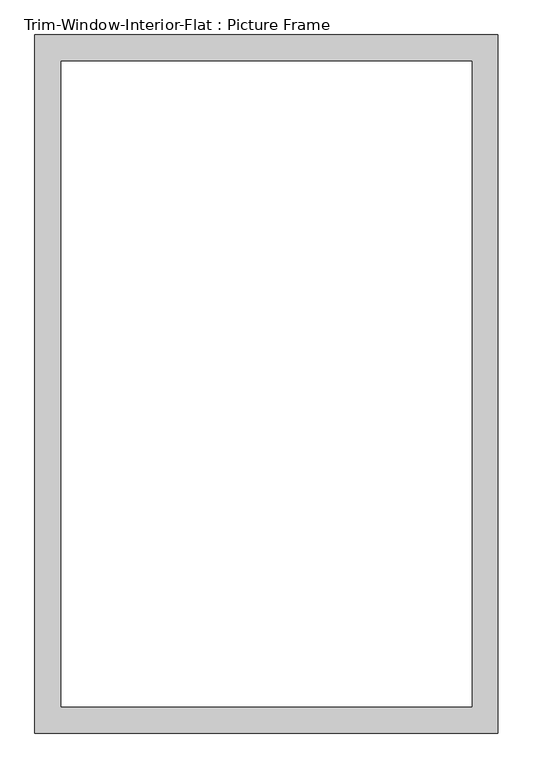
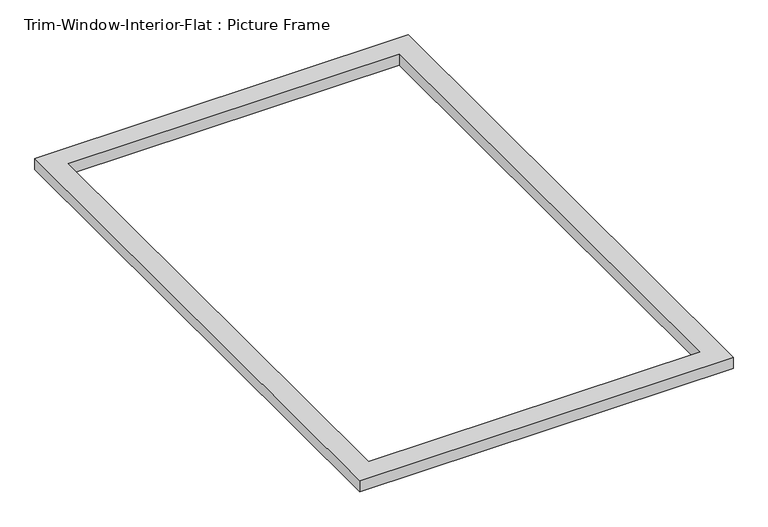
"""IFC4 building model written with IfcOpenShell, lengths in millimetres: proxy geometry, Trim-Window-Interior-Flat : Picture Frame."""

import ifcopenshell
import ifcopenshell.guid

model = None  # the IFC model being written
_history = None  # IfcOwnerHistory: only IFC2X3 demands one
_inside = {}  # id of a spatial element -> (the spatial element, [elements in it])
_under = {}  # id of a project, library or spatial element -> (it, [spatial elements below it])
_declared = {}  # id of a project -> (the project, [libraries it declares])
_typed = {}  # id of a type object -> (the type object, [elements of that type])
_made_of = {}  # id of a material, layer set ... -> (it, [elements and type objects made of it])


def new_model(schema):
    """Start an empty IFC model of exactly this schema.

    Asked for "IFC4X3", IfcOpenShell would pick the latest addendum, in which some entities
    have other attributes; the version numbers below select the first issue.
    IFC2X3 requires an IfcOwnerHistory on every rooted entity: one is made here for all.
    """
    global model, _history
    if schema == "IFC4X3":
        model = ifcopenshell.file(schema_version=(4, 3, 0, 0))
    else:
        model = ifcopenshell.file(schema=schema)
    _inside.clear()
    _under.clear()
    _declared.clear()
    _typed.clear()
    _made_of.clear()
    _history = None
    if model.schema == "IFC2X3":
        org = make("IfcOrganization", Name="unknown")
        user = make(
            "IfcPersonAndOrganization",
            ThePerson=make("IfcPerson", FamilyName="unknown"),
            TheOrganization=org,
        )
        app = make(
            "IfcApplication",
            ApplicationDeveloper=org,
            Version="unknown",
            ApplicationFullName="unknown",
            ApplicationIdentifier="unknown",
        )
        _history = make(
            "IfcOwnerHistory",
            OwningUser=user,
            OwningApplication=app,
            ChangeAction="ADDED",
            CreationDate=0,
        )
    return model


def make(cls, **values):
    """One entity of the class cls with the attributes given. An attribute that is None is left unset."""
    return model.create_entity(
        cls, **{name: value for name, value in values.items() if value is not None}
    )


def rooted(cls, **values):
    """An entity with a GlobalId (a new one), such as an element, a storey or a relation."""
    return make(cls, GlobalId=ifcopenshell.guid.new(), OwnerHistory=_history, **values)


def si_unit(unit_type, name, prefix=None):
    """IfcSIUnit, for example si_unit("LENGTHUNIT", "METRE", prefix="MILLI")."""
    return make("IfcSIUnit", UnitType=unit_type, Prefix=prefix, Name=name)


def assignment(units):
    """IfcUnitAssignment: the units of a project."""
    return None if units is None else make("IfcUnitAssignment", Units=units)


def point(xyz):
    """IfcCartesianPoint."""
    return None if xyz is None else make("IfcCartesianPoint", Coordinates=xyz)


def direction(xyz):
    """IfcDirection."""
    return None if xyz is None else make("IfcDirection", DirectionRatios=xyz)


def frame(location, z_axis=None, x_axis=None):
    """IfcAxis2Placement3D, a coordinate frame: its origin and axes. An axis left out is left unset."""
    return make(
        "IfcAxis2Placement3D",
        Location=point(location),
        Axis=direction(z_axis),
        RefDirection=direction(x_axis),
    )


def origin():
    """The frame at (0, 0, 0) with its axes left unset."""
    return frame((0.0, 0.0, 0.0))


def origin_with_axes():
    """The frame at (0, 0, 0) with the z axis (0, 0, 1) and the x axis (1, 0, 0) written out."""
    return frame((0.0, 0.0, 0.0), z_axis=(0.0, 0.0, 1.0), x_axis=(1.0, 0.0, 0.0))


def place(relative_to, where):
    """IfcLocalPlacement: puts the frame where relative to a parent placement (None: the world)."""
    return make(
        "IfcLocalPlacement", PlacementRelTo=relative_to, RelativePlacement=where
    )


def context(
    kind, dimensions, precision=None, world=None, true_north=None, identifier=None
):
    """IfcGeometricRepresentationContext, for example the 3D "Model" context."""
    return make(
        "IfcGeometricRepresentationContext",
        ContextIdentifier=identifier,
        ContextType=kind,
        CoordinateSpaceDimension=dimensions,
        Precision=precision,
        WorldCoordinateSystem=world,
        TrueNorth=true_north,
    )


def project(units=None, contexts=None):
    """IfcProject with its units and contexts."""
    return rooted(
        "IfcProject",
        Name="project",
        RepresentationContexts=contexts,
        UnitsInContext=assignment(units),
    )


def spatial(cls, under=None, at=None, **own):
    """A site, building, storey or space (cls), placed at a placement, below another one or the project."""
    s = rooted(cls, ObjectPlacement=at, **own)
    if under is not None:
        _under.setdefault(under.id(), (under, []))[1].append(s)
    return s


def polyline(points):
    """IfcPolyline through the points."""
    return make("IfcPolyline", Points=[point(p) for p in points])


def outline(outer, holes=None, kind="AREA"):
    """IfcArbitraryClosedProfileDef: a profile drawn as a closed curve; with holes, ...WithVoids."""
    if holes is None:
        return make("IfcArbitraryClosedProfileDef", ProfileType=kind, OuterCurve=outer)
    return make(
        "IfcArbitraryProfileDefWithVoids",
        ProfileType=kind,
        OuterCurve=outer,
        InnerCurves=holes,
    )


def extrude(swept, where, along, depth):
    """IfcExtrudedAreaSolid: the profile swept, set in the frame where, extruded along a direction by depth."""
    return make(
        "IfcExtrudedAreaSolid",
        SweptArea=swept,
        Position=where,
        ExtrudedDirection=direction(along),
        Depth=depth,
    )


def shape(context_of_items, identifier, shape_type, items):
    """IfcShapeRepresentation: the items that make up one representation, for example the "Body"."""
    return make(
        "IfcShapeRepresentation",
        ContextOfItems=context_of_items,
        RepresentationIdentifier=identifier,
        RepresentationType=shape_type,
        Items=items,
    )


def source(mapping_origin, context_of_items, identifier, shape_type, items):
    """IfcRepresentationMap: a shape defined once, which mapped items show again and again."""
    return make(
        "IfcRepresentationMap",
        MappingOrigin=mapping_origin,
        MappedRepresentation=shape(context_of_items, identifier, shape_type, items),
    )


def transform(
    local_origin,
    x_axis=None,
    y_axis=None,
    z_axis=None,
    scale=None,
    scale2=None,
    scale3=None,
    uniform=True,
):
    """IfcCartesianTransformationOperator3D, or its non-uniform kind. x_axis, y_axis, z_axis: its Axis1, 2, 3."""
    if uniform:
        return make(
            "IfcCartesianTransformationOperator3D",
            Axis1=direction(x_axis),
            Axis2=direction(y_axis),
            LocalOrigin=point(local_origin),
            Scale=scale,
            Axis3=direction(z_axis),
        )
    return make(
        "IfcCartesianTransformationOperator3DnonUniform",
        Axis1=direction(x_axis),
        Axis2=direction(y_axis),
        LocalOrigin=point(local_origin),
        Scale=scale,
        Axis3=direction(z_axis),
        Scale2=scale2,
        Scale3=scale3,
    )


def mapped(mapping_source, mapping_target):
    """IfcMappedItem: shows the shape of a source again, moved by a transform."""
    return make(
        "IfcMappedItem", MappingSource=mapping_source, MappingTarget=mapping_target
    )


def made_of(thing, what):
    """Note that an element or type object is made of a material, layer set ...; save() writes the relation."""
    if what is not None:
        _made_of.setdefault(what.id(), (what, []))[1].append(thing)
    return thing


def element(
    cls,
    number,
    at=None,
    inside=None,
    cuts=None,
    type_object=None,
    material=None,
    context=None,
    identifier="Body",
    shape_type=None,
    held_by="IfcProductDefinitionShape",
    body=None,
    shapes=None,
    **own,
):
    """One element of the class cls, such as IfcWall. Its Tag is "e" and its number.

    at: its placement. inside: the storey or other place that contains it. cuts: it is an
    opening in that element (IfcRelVoidsElement). A single representation is given by context,
    identifier, shape_type and body (its items); several are given by shapes. held_by: the class
    of the entity that holds the representations. save() writes the other relations.
    """
    e = rooted(cls, Tag="e%d" % number, ObjectPlacement=at, **own)
    if body is not None:
        shapes = [shape(context, identifier, shape_type, body)]
    if shapes is not None:
        e.Representation = make(held_by, Representations=shapes)
    if inside is not None:
        _inside.setdefault(inside.id(), (inside, []))[1].append(e)
    if cuts is not None:
        rooted(
            "IfcRelVoidsElement", RelatingBuildingElement=cuts, RelatedOpeningElement=e
        )
    if type_object is not None:
        _typed.setdefault(type_object.id(), (type_object, []))[1].append(e)
    return made_of(e, material)


def aggregate(whole, parts):
    """IfcRelAggregates: a whole, such as a stair, and the parts it consists of."""
    return rooted("IfcRelAggregates", RelatingObject=whole, RelatedObjects=parts)


def save(model, path):
    """Write the relations noted so far, then the file.

    IfcRelAggregates (storeys below a building ...), IfcRelContainedInSpatialStructure (elements
    in a storey), IfcRelDefinesByType, IfcRelAssociatesMaterial and IfcRelDeclares: one each for
    every whole, place, type object, material and project.
    """
    for whole, parts in _under.values():
        aggregate(whole, parts)
    for where, things in _inside.values():
        rooted(
            "IfcRelContainedInSpatialStructure",
            RelatedElements=things,
            RelatingStructure=where,
        )
    for kind, things in _typed.values():
        rooted("IfcRelDefinesByType", RelatedObjects=things, RelatingType=kind)
    for what, things in _made_of.values():
        rooted("IfcRelAssociatesMaterial", RelatedObjects=things, RelatingMaterial=what)
    for by, libraries in _declared.values():
        rooted("IfcRelDeclares", RelatingContext=by, RelatedDefinitions=libraries)
    model.write(path)


def trim_window_interior_flat_picture_frame_b9635a36(model_context):
    return source(origin(), model_context, "Body", "SweptSolid", [
        extrude(outline(polyline([(501.65, -44.45), (-501.65, -44.45), (-501.65, 1466.85), (501.65, 1466.85), (501.65, -44.45)]), holes=[polyline([(444.5, 12.7), (444.5, 1409.7), (-444.5, 1409.7), (-444.5, 12.7), (444.5, 12.7)])]), origin_with_axes(), (0.0, 0.0, 1.0), 31.75),
    ])


if __name__ == "__main__":
    model = new_model("IFC4")
    model_context = context("Model", 3, world=origin())
    ifc_project = project(units=[si_unit("LENGTHUNIT", "METRE", prefix="MILLI")], contexts=[model_context])
    site = spatial("IfcSite", under=ifc_project)
    building = spatial("IfcBuilding", under=site)
    placement = place(None, origin())
    trim_window_interior_flat_picture_frame_shape = trim_window_interior_flat_picture_frame_b9635a36(model_context)
    element("IfcBuildingElementProxy", 1, Name="Trim-Window-Interior-Flat : Picture Frame", ObjectType="Trim-Window-Interior-Flat : Picture Frame", at=placement, inside=building, context=model_context, shape_type="MappedRepresentation", body=[
        mapped(trim_window_interior_flat_picture_frame_shape, transform((0.0, 0.0, 0.0), x_axis=(1.0, 0.0, 0.0), y_axis=(0.0, 1.0, 0.0), z_axis=(0.0, 0.0, 1.0))),
    ])
    save(model, "model.ifc")

# Revit data of these elements
# Type "Trim-Window-Interior-Flat : Picture Frame"
#   Trim Thickness_Picture Frame = 0' - 1 1/4"
#   Trim Width = 0' - 2 1/4"
#   Trim Thickness_with Sill = 0' - 0 3/4"
#   Sill Thickness = 0' - 1 1/4"
#   Opening Width [instance default] = 2' - 0"
#   Opening Height [instance default] = 3' - 0"
#   Default Elevation = 4' - 0"
#   Sill = no
#   Picture Frame = yes
#   Trim Material [instance default] = none
# Element 1 (IfcBuildingElementProxy, "Trim-Window-Interior-Flat : Picture Frame")
#   Opening Width = 3' - 0"
#   Opening Height = 4' - 8"
#   Trim Material = Wood - Stained
#   Materials on its faces: "Wood - Stained"
# Materials
#   "Wood - Stained": class "Wood", colour RGB 224 178 126, transparency 0, Cost = 0
